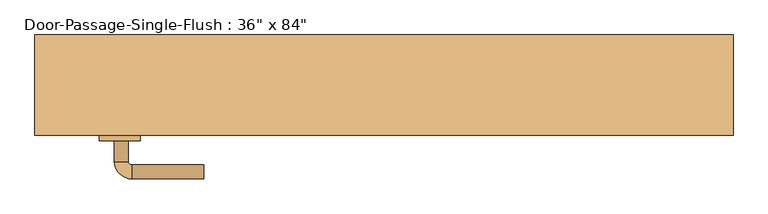
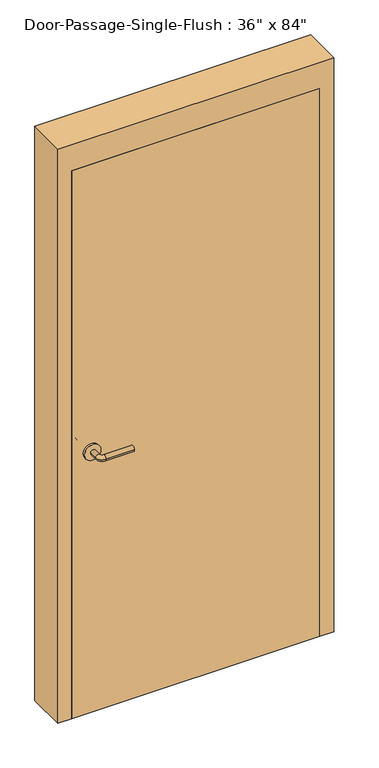
"""IFC4 building model written with IfcOpenShell, lengths in millimetres: door geometry."""

import ifcopenshell
import ifcopenshell.guid

model = None  # the IFC model being written
_history = None  # IfcOwnerHistory: only IFC2X3 demands one
_inside = {}  # id of a spatial element -> (the spatial element, [elements in it])
_under = {}  # id of a project, library or spatial element -> (it, [spatial elements below it])
_declared = {}  # id of a project -> (the project, [libraries it declares])
_typed = {}  # id of a type object -> (the type object, [elements of that type])
_made_of = {}  # id of a material, layer set ... -> (it, [elements and type objects made of it])


def new_model(schema):
    """Start an empty IFC model of exactly this schema.

    Asked for "IFC4X3", IfcOpenShell would pick the latest addendum, in which some entities
    have other attributes; the version numbers below select the first issue.
    IFC2X3 requires an IfcOwnerHistory on every rooted entity: one is made here for all.
    """
    global model, _history
    if schema == "IFC4X3":
        model = ifcopenshell.file(schema_version=(4, 3, 0, 0))
    else:
        model = ifcopenshell.file(schema=schema)
    _inside.clear()
    _under.clear()
    _declared.clear()
    _typed.clear()
    _made_of.clear()
    _history = None
    if model.schema == "IFC2X3":
        org = make("IfcOrganization", Name="unknown")
        user = make(
            "IfcPersonAndOrganization",
            ThePerson=make("IfcPerson", FamilyName="unknown"),
            TheOrganization=org,
        )
        app = make(
            "IfcApplication",
            ApplicationDeveloper=org,
            Version="unknown",
            ApplicationFullName="unknown",
            ApplicationIdentifier="unknown",
        )
        _history = make(
            "IfcOwnerHistory",
            OwningUser=user,
            OwningApplication=app,
            ChangeAction="ADDED",
            CreationDate=0,
        )
    return model


def make(cls, **values):
    """One entity of the class cls with the attributes given. An attribute that is None is left unset."""
    return model.create_entity(
        cls, **{name: value for name, value in values.items() if value is not None}
    )


def rooted(cls, **values):
    """An entity with a GlobalId (a new one), such as an element, a storey or a relation."""
    return make(cls, GlobalId=ifcopenshell.guid.new(), OwnerHistory=_history, **values)


def si_unit(unit_type, name, prefix=None):
    """IfcSIUnit, for example si_unit("LENGTHUNIT", "METRE", prefix="MILLI")."""
    return make("IfcSIUnit", UnitType=unit_type, Prefix=prefix, Name=name)


def assignment(units):
    """IfcUnitAssignment: the units of a project."""
    return None if units is None else make("IfcUnitAssignment", Units=units)


def point(xyz):
    """IfcCartesianPoint."""
    return None if xyz is None else make("IfcCartesianPoint", Coordinates=xyz)


def direction(xyz):
    """IfcDirection."""
    return None if xyz is None else make("IfcDirection", DirectionRatios=xyz)


def frame(location, z_axis=None, x_axis=None):
    """IfcAxis2Placement3D, a coordinate frame: its origin and axes. An axis left out is left unset."""
    return make(
        "IfcAxis2Placement3D",
        Location=point(location),
        Axis=direction(z_axis),
        RefDirection=direction(x_axis),
    )


def frame_2d(location, x_axis=None):
    """IfcAxis2Placement2D, a coordinate frame in the plane: its origin and x axis."""
    return make(
        "IfcAxis2Placement2D", Location=point(location), RefDirection=direction(x_axis)
    )


def origin():
    """The frame at (0, 0, 0) with its axes left unset."""
    return frame((0.0, 0.0, 0.0))


def origin_with_axes():
    """The frame at (0, 0, 0) with the z axis (0, 0, 1) and the x axis (1, 0, 0) written out."""
    return frame((0.0, 0.0, 0.0), z_axis=(0.0, 0.0, 1.0), x_axis=(1.0, 0.0, 0.0))


def place(relative_to, where):
    """IfcLocalPlacement: puts the frame where relative to a parent placement (None: the world)."""
    return make(
        "IfcLocalPlacement", PlacementRelTo=relative_to, RelativePlacement=where
    )


def context(
    kind, dimensions, precision=None, world=None, true_north=None, identifier=None
):
    """IfcGeometricRepresentationContext, for example the 3D "Model" context."""
    return make(
        "IfcGeometricRepresentationContext",
        ContextIdentifier=identifier,
        ContextType=kind,
        CoordinateSpaceDimension=dimensions,
        Precision=precision,
        WorldCoordinateSystem=world,
        TrueNorth=true_north,
    )


def project(units=None, contexts=None):
    """IfcProject with its units and contexts."""
    return rooted(
        "IfcProject",
        Name="project",
        RepresentationContexts=contexts,
        UnitsInContext=assignment(units),
    )


def spatial(cls, under=None, at=None, **own):
    """A site, building, storey or space (cls), placed at a placement, below another one or the project."""
    s = rooted(cls, ObjectPlacement=at, **own)
    if under is not None:
        _under.setdefault(under.id(), (under, []))[1].append(s)
    return s


def polyline(points):
    """IfcPolyline through the points."""
    return make("IfcPolyline", Points=[point(p) for p in points])


def circle_curve(where, radius):
    """IfcCircle in the frame where."""
    return make("IfcCircle", Position=where, Radius=radius)


def ellipse_curve(where, semi_axis1, semi_axis2):
    """IfcEllipse in the frame where."""
    return make(
        "IfcEllipse", Position=where, SemiAxis1=semi_axis1, SemiAxis2=semi_axis2
    )


def trimmed(basis, trim1, trim2, sense, master):
    """IfcTrimmedCurve: the piece of a basis curve between two trims."""
    return make(
        "IfcTrimmedCurve",
        BasisCurve=basis,
        Trim1=trim1,
        Trim2=trim2,
        SenseAgreement=sense,
        MasterRepresentation=master,
    )


def segment(curve, same_sense, transition):
    """IfcCompositeCurveSegment."""
    return make(
        "IfcCompositeCurveSegment",
        Transition=transition,
        SameSense=same_sense,
        ParentCurve=curve,
    )


def composite_curve(segments, self_intersect=None):
    """IfcCompositeCurve: segments joined end to end."""
    return make("IfcCompositeCurve", Segments=segments, SelfIntersect=self_intersect)


def outline(outer, holes=None, kind="AREA"):
    """IfcArbitraryClosedProfileDef: a profile drawn as a closed curve; with holes, ...WithVoids."""
    if holes is None:
        return make("IfcArbitraryClosedProfileDef", ProfileType=kind, OuterCurve=outer)
    return make(
        "IfcArbitraryProfileDefWithVoids",
        ProfileType=kind,
        OuterCurve=outer,
        InnerCurves=holes,
    )


def extrude(swept, where, along, depth):
    """IfcExtrudedAreaSolid: the profile swept, set in the frame where, extruded along a direction by depth."""
    return make(
        "IfcExtrudedAreaSolid",
        SweptArea=swept,
        Position=where,
        ExtrudedDirection=direction(along),
        Depth=depth,
    )


def faces_of(points, faces, orient=None, outer=None):
    """IfcFace entities. A face is a list of loops; a loop is a list of indices into points, from 0.

    orient and outer hold one flag for each loop. By default every Orientation is true, the
    first loop of a face is its IfcFaceOuterBound and the others are IfcFaceBound.
    """
    made = []
    for i, loops in enumerate(faces):
        bounds = []
        for j, loop in enumerate(loops):
            is_outer = j == 0 if outer is None else outer[i][j]
            bounds.append(
                make(
                    "IfcFaceOuterBound" if is_outer else "IfcFaceBound",
                    Bound=make("IfcPolyLoop", Polygon=[points[k] for k in loop]),
                    Orientation=True if orient is None else orient[i][j],
                )
            )
        made.append(make("IfcFace", Bounds=bounds))
    return made


def faceted_brep(points, faces, orient=None, outer=None, voids=None):
    """IfcFacetedBrep: a solid bounded by flat faces; with voids (closed shells), ...WithVoids."""
    shared = [point(p) for p in points]
    hull = make("IfcClosedShell", CfsFaces=faces_of(shared, faces, orient, outer))
    if voids is None:
        return make("IfcFacetedBrep", Outer=hull)
    return make(
        "IfcFacetedBrepWithVoids",
        Outer=hull,
        Voids=[
            make(cls, CfsFaces=faces_of(shared, fs, o, b)) for cls, fs, o, b in voids
        ],
    )


def shape(context_of_items, identifier, shape_type, items):
    """IfcShapeRepresentation: the items that make up one representation, for example the "Body"."""
    return make(
        "IfcShapeRepresentation",
        ContextOfItems=context_of_items,
        RepresentationIdentifier=identifier,
        RepresentationType=shape_type,
        Items=items,
    )


def source(mapping_origin, context_of_items, identifier, shape_type, items):
    """IfcRepresentationMap: a shape defined once, which mapped items show again and again."""
    return make(
        "IfcRepresentationMap",
        MappingOrigin=mapping_origin,
        MappedRepresentation=shape(context_of_items, identifier, shape_type, items),
    )


def transform(
    local_origin,
    x_axis=None,
    y_axis=None,
    z_axis=None,
    scale=None,
    scale2=None,
    scale3=None,
    uniform=True,
):
    """IfcCartesianTransformationOperator3D, or its non-uniform kind. x_axis, y_axis, z_axis: its Axis1, 2, 3."""
    if uniform:
        return make(
            "IfcCartesianTransformationOperator3D",
            Axis1=direction(x_axis),
            Axis2=direction(y_axis),
            LocalOrigin=point(local_origin),
            Scale=scale,
            Axis3=direction(z_axis),
        )
    return make(
        "IfcCartesianTransformationOperator3DnonUniform",
        Axis1=direction(x_axis),
        Axis2=direction(y_axis),
        LocalOrigin=point(local_origin),
        Scale=scale,
        Axis3=direction(z_axis),
        Scale2=scale2,
        Scale3=scale3,
    )


def mapped(mapping_source, mapping_target):
    """IfcMappedItem: shows the shape of a source again, moved by a transform."""
    return make(
        "IfcMappedItem", MappingSource=mapping_source, MappingTarget=mapping_target
    )


def made_of(thing, what):
    """Note that an element or type object is made of a material, layer set ...; save() writes the relation."""
    if what is not None:
        _made_of.setdefault(what.id(), (what, []))[1].append(thing)
    return thing


def element(
    cls,
    number,
    at=None,
    inside=None,
    cuts=None,
    type_object=None,
    material=None,
    context=None,
    identifier="Body",
    shape_type=None,
    held_by="IfcProductDefinitionShape",
    body=None,
    shapes=None,
    **own,
):
    """One element of the class cls, such as IfcWall. Its Tag is "e" and its number.

    at: its placement. inside: the storey or other place that contains it. cuts: it is an
    opening in that element (IfcRelVoidsElement). A single representation is given by context,
    identifier, shape_type and body (its items); several are given by shapes. held_by: the class
    of the entity that holds the representations. save() writes the other relations.
    """
    e = rooted(cls, Tag="e%d" % number, ObjectPlacement=at, **own)
    if body is not None:
        shapes = [shape(context, identifier, shape_type, body)]
    if shapes is not None:
        e.Representation = make(held_by, Representations=shapes)
    if inside is not None:
        _inside.setdefault(inside.id(), (inside, []))[1].append(e)
    if cuts is not None:
        rooted(
            "IfcRelVoidsElement", RelatingBuildingElement=cuts, RelatedOpeningElement=e
        )
    if type_object is not None:
        _typed.setdefault(type_object.id(), (type_object, []))[1].append(e)
    return made_of(e, material)


def aggregate(whole, parts):
    """IfcRelAggregates: a whole, such as a stair, and the parts it consists of."""
    return rooted("IfcRelAggregates", RelatingObject=whole, RelatedObjects=parts)


def save(model, path):
    """Write the relations noted so far, then the file.

    IfcRelAggregates (storeys below a building ...), IfcRelContainedInSpatialStructure (elements
    in a storey), IfcRelDefinesByType, IfcRelAssociatesMaterial and IfcRelDeclares: one each for
    every whole, place, type object, material and project.
    """
    for whole, parts in _under.values():
        aggregate(whole, parts)
    for where, things in _inside.values():
        rooted(
            "IfcRelContainedInSpatialStructure",
            RelatedElements=things,
            RelatingStructure=where,
        )
    for kind, things in _typed.values():
        rooted("IfcRelDefinesByType", RelatedObjects=things, RelatingType=kind)
    for what, things in _made_of.values():
        rooted("IfcRelAssociatesMaterial", RelatedObjects=things, RelatingMaterial=what)
    for by, libraries in _declared.values():
        rooted("IfcRelDeclares", RelatingContext=by, RelatedDefinitions=libraries)
    model.write(path)


def plane_surface(at):
    """IfcPlane: the flat surface through the origin of the frame at, square to its z axis."""
    return make("IfcPlane", Position=at)


def cylinder_surface(at, radius):
    """IfcCylindricalSurface: all points at the distance radius from the z axis of the frame at."""
    return make("IfcCylindricalSurface", Position=at, Radius=radius)


def revolved_surface(curve, axis_point, axis_direction):
    """IfcSurfaceOfRevolution: the curve turned about the line through axis_point along axis_direction."""
    return make(
        "IfcSurfaceOfRevolution",
        SweptCurve=make("IfcArbitraryOpenProfileDef", ProfileType="CURVE", Curve=curve),
        AxisPosition=make("IfcAxis1Placement", Location=point(axis_point), Axis=direction(axis_direction)),
    )


def advanced_brep(points, edges, surfaces, faces):
    """IfcAdvancedBrep: a solid bounded by faces that lie on surfaces and meet in shared edges.

    An edge is (start, end): straight between two places in points (the first is 0);
    or (start, end, curve); or (start, end, curve, False) where it runs against its curve.
    A face is (place in surfaces, loops), or (place, loops, False) where it looks against
    its surface's normal. A loop lists edges by number (the first is 1), with a minus sign
    where the edge is run from its end to its start. The first loop is the outer one.
    """
    corners = [point(p) for p in points]
    vertices = [make("IfcVertexPoint", VertexGeometry=c) for c in corners]
    made = []
    for start, end, *more in edges:
        made.append(
            make(
                "IfcEdgeCurve",
                EdgeStart=vertices[start],
                EdgeEnd=vertices[end],
                EdgeGeometry=more[0] if more else make("IfcPolyline", Points=[corners[start], corners[end]]),
                SameSense=more[1] if len(more) > 1 else True,
            )
        )
    hull = []
    for where, loops, *sense in faces:
        bounds = []
        for j, loop in enumerate(loops):
            ring = [make("IfcOrientedEdge", EdgeElement=made[abs(k) - 1], Orientation=k > 0) for k in loop]
            bounds.append(
                make(
                    "IfcFaceOuterBound" if j == 0 else "IfcFaceBound",
                    Bound=make("IfcEdgeLoop", EdgeList=ring),
                    Orientation=True,
                )
            )
        hull.append(make("IfcAdvancedFace", Bounds=bounds, FaceSurface=surfaces[where], SameSense=sense[0] if sense else True))
    return make("IfcAdvancedBrep", Outer=make("IfcClosedShell", CfsFaces=hull))


def door_58febf71(model_context):
    return source(origin(), model_context, "Body", "SolidModel", [
        advanced_brep(
        [(-392.190625, -76.1375, 1016.0), (-372.190625, -76.1375, 1016.0), (-392.190625, -46.1375, 1016.0), (-372.190625, -46.1375, 1016.0), (-367.190625, -41.1375, 1016.0), (-367.190625, -21.1375, 1016.0), (-262.190625, -21.1375, 1016.0), (-262.190625, -41.1375, 1016.0)],
        [
            (0, 1, circle_curve(frame((-382.190625, -76.1375, 1016.0), z_axis=(0.0, -1.0, 0.0), x_axis=(1.0, 0.0, 0.0)), 10.0)),
            (1, 0, circle_curve(frame((-382.190625, -76.1375, 1016.0), z_axis=(0.0, -1.0, 0.0), x_axis=(1.0, 0.0, 0.0)), 10.0)),
            (0, 2),
            (2, 3, circle_curve(frame((-382.190625, -46.1375, 1016.0), z_axis=(0.0, -1.0, 0.0), x_axis=(1.0, 0.0, 0.0)), 10.0)),
            (3, 1),
            (3, 2, circle_curve(frame((-382.190625, -46.1375, 1016.0), z_axis=(0.0, -1.0, 0.0), x_axis=(1.0, 0.0, 0.0)), 10.0)),
            (4, 3, circle_curve(frame((-367.190625, -46.1375, 1016.0), z_axis=(0.0, 0.0, 1.0), x_axis=(-1.0, 0.0, 0.0)), 5.0)),
            (2, 5, circle_curve(frame((-367.190625, -46.1375, 1016.0), z_axis=(0.0, 0.0, -1.0), x_axis=(-1.0, 0.0, 0.0)), 25.0)),
            (5, 4, circle_curve(frame((-367.190625, -31.1375, 1016.0), z_axis=(-1.0, 0.0, 0.0), x_axis=(0.0, -1.0, 0.0)), 10.0)),
            (4, 5, circle_curve(frame((-367.190625, -31.1375, 1016.0), z_axis=(-1.0, 0.0, 0.0), x_axis=(0.0, -1.0, 0.0)), 10.0)),
            (6, 7, circle_curve(frame((-262.190625, -31.1375, 1016.0), z_axis=(1.0, 0.0, 0.0), x_axis=(0.0, -1.0, 0.0)), 10.0)),
            (7, 6, circle_curve(frame((-262.190625, -31.1375, 1016.0), z_axis=(1.0, 0.0, 0.0), x_axis=(0.0, -1.0, 0.0)), 10.0)),
            (5, 6),
            (7, 4),
        ],
        [
            plane_surface(frame((-382.190625, -76.1375, 1016.0), z_axis=(0.0, -1.0, 0.0), x_axis=(0.0, 0.0, 1.0))),
            cylinder_surface(frame((-382.190625, -76.1375, 1016.0), z_axis=(0.0, -1.0, 0.0), x_axis=(1.0, 0.0, 0.0)), 10.0),
            revolved_surface(trimmed(ellipse_curve(frame((-382.190625, -46.1375, 1016.0), z_axis=(0.0, -1.0, 0.0), x_axis=(1.0, 0.0, 0.0)), 10.0, 10.0), [point((-392.190625, -46.1375, 1016.0))], [point((-372.190625, -46.1375, 1016.0))], True, "CARTESIAN"), (-367.190625, -46.1375, 1016.0), (0.0, 0.0, -1.0)),
            revolved_surface(trimmed(ellipse_curve(frame((-382.190625, -46.1375, 1016.0), z_axis=(0.0, -1.0, 0.0), x_axis=(1.0, 0.0, 0.0)), 10.0, 10.0), [point((-372.190625, -46.1375, 1016.0))], [point((-392.190625, -46.1375, 1016.0))], True, "CARTESIAN"), (-367.190625, -46.1375, 1016.0), (0.0, 0.0, -1.0)),
            plane_surface(frame((-262.190625, -31.1375, 1016.0), z_axis=(1.0, 0.0, 0.0), x_axis=(0.0, 0.0, 1.0))),
            cylinder_surface(frame((-367.190625, -31.1375, 1016.0), z_axis=(-1.0, 0.0, 0.0), x_axis=(0.0, -1.0, 0.0)), 10.0),
        ],
        [
            (0, [[1, 2]]),
            (1, [[-1, 3, 4, 5]]),
            (1, [[-2, -5, 6, -3]]),
            (2, [[7, -4, 8, 9]]),
            (3, [[-8, -6, -7, 10]]),
            (4, [[11, 12]]),
            (5, [[-9, 13, -12, 14]]),
            (5, [[-10, -14, -11, -13]]),
        ],
    ),
        extrude(outline(composite_curve([segment(trimmed(circle_curve(frame_2d((1016.0, -384.690625)), 30.0), [point((1016.0, -414.690625))], [point((1016.0, -354.690625))], False, "CARTESIAN"), True, "CONTINUOUS"), segment(trimmed(circle_curve(frame_2d((1016.0, -384.690625)), 30.0), [point((1016.0, -354.690625))], [point((1016.0, -414.690625))], False, "CARTESIAN"), True, "CONTINUOUS")], self_intersect=False)), frame((0.0, -84.1375, 0.0), z_axis=(0.0, 1.0, 0.0), x_axis=(0.0, 0.0, 1.0)), (0.0, 0.0, 1.0), 8.0),
        advanced_brep(
        [(-392.190625, -136.5875, 1016.0), (-372.190625, -136.5875, 1016.0), (-372.190625, -166.5875, 1016.0), (-392.190625, -166.5875, 1016.0), (-367.190625, -171.5875, 1016.0), (-367.190625, -191.5875, 1016.0), (-262.190625, -191.5875, 1016.0), (-262.190625, -171.5875, 1016.0)],
        [
            (0, 1, circle_curve(frame((-382.190625, -136.5875, 1016.0), z_axis=(0.0, 1.0, 0.0), x_axis=(1.0, 0.0, 0.0)), 10.0)),
            (1, 0, circle_curve(frame((-382.190625, -136.5875, 1016.0), z_axis=(0.0, 1.0, 0.0), x_axis=(1.0, 0.0, 0.0)), 10.0)),
            (1, 2),
            (2, 3, circle_curve(frame((-382.190625, -166.5875, 1016.0), z_axis=(0.0, 1.0, 0.0), x_axis=(1.0, 0.0, 0.0)), 10.0)),
            (3, 0),
            (3, 2, circle_curve(frame((-382.190625, -166.5875, 1016.0), z_axis=(0.0, 1.0, 0.0), x_axis=(1.0, 0.0, 0.0)), 10.0)),
            (4, 5, circle_curve(frame((-367.190625, -181.5875, 1016.0), z_axis=(-1.0, 0.0, 0.0), x_axis=(0.0, 1.0, 0.0)), 10.0)),
            (5, 3, circle_curve(frame((-367.190625, -166.5875, 1016.0), z_axis=(0.0, 0.0, -1.0), x_axis=(-1.0, 0.0, 0.0)), 25.0)),
            (2, 4, circle_curve(frame((-367.190625, -166.5875, 1016.0), z_axis=(0.0, 0.0, 1.0), x_axis=(-1.0, 0.0, 0.0)), 5.0)),
            (5, 4, circle_curve(frame((-367.190625, -181.5875, 1016.0), z_axis=(-1.0, 0.0, 0.0), x_axis=(0.0, 1.0, 0.0)), 10.0)),
            (6, 7, circle_curve(frame((-262.190625, -181.5875, 1016.0), z_axis=(1.0, 0.0, 0.0), x_axis=(0.0, 1.0, 0.0)), 10.0)),
            (7, 6, circle_curve(frame((-262.190625, -181.5875, 1016.0), z_axis=(1.0, 0.0, 0.0), x_axis=(0.0, 1.0, 0.0)), 10.0)),
            (4, 7),
            (6, 5),
        ],
        [
            plane_surface(frame((-382.190625, -136.5875, 1016.0), z_axis=(0.0, 1.0, 0.0), x_axis=(0.0, 0.0, 1.0))),
            cylinder_surface(frame((-382.190625, -136.5875, 1016.0), z_axis=(0.0, 1.0, 0.0), x_axis=(1.0, 0.0, 0.0)), 10.0),
            revolved_surface(trimmed(ellipse_curve(frame((-382.190625, -166.5875, 1016.0), z_axis=(0.0, -1.0, 0.0), x_axis=(1.0, 0.0, 0.0)), 10.0, 10.0), [point((-392.190625, -166.5875, 1016.0))], [point((-372.190625, -166.5875, 1016.0))], True, "CARTESIAN"), (-367.190625, -166.5875, 1016.0), (0.0, 0.0, -1.0)),
            revolved_surface(trimmed(ellipse_curve(frame((-382.190625, -166.5875, 1016.0), z_axis=(0.0, -1.0, 0.0), x_axis=(1.0, 0.0, 0.0)), 10.0, 10.0), [point((-372.190625, -166.5875, 1016.0))], [point((-392.190625, -166.5875, 1016.0))], True, "CARTESIAN"), (-367.190625, -166.5875, 1016.0), (0.0, 0.0, -1.0)),
            plane_surface(frame((-262.190625, -181.5875, 1016.0), z_axis=(1.0, 0.0, 0.0), x_axis=(0.0, 0.0, 1.0))),
            cylinder_surface(frame((-367.190625, -181.5875, 1016.0), z_axis=(-1.0, 0.0, 0.0), x_axis=(0.0, 1.0, 0.0)), 10.0),
        ],
        [
            (0, [[1, 2]]),
            (1, [[3, 4, 5, -2]]),
            (1, [[-5, 6, -3, -1]]),
            (2, [[7, 8, -4, 9]]),
            (3, [[10, -9, -6, -8]]),
            (4, [[11, 12]]),
            (5, [[13, -11, 14, -7]]),
            (5, [[-14, -12, -13, -10]]),
        ],
    ),
        extrude(outline(composite_curve([segment(trimmed(circle_curve(frame_2d((1016.0, -384.690625)), 30.0), [point((1016.0, -414.690625))], [point((1016.0, -354.690625))], False, "CARTESIAN"), True, "CONTINUOUS"), segment(trimmed(circle_curve(frame_2d((1016.0, -384.690625)), 30.0), [point((1016.0, -354.690625))], [point((1016.0, -414.690625))], False, "CARTESIAN"), True, "CONTINUOUS")], self_intersect=False)), frame((0.0, -136.5875, 0.0), z_axis=(0.0, 1.0, 0.0), x_axis=(0.0, 0.0, 1.0)), (0.0, 0.0, 1.0), 8.0),
        faceted_brep([(457.2, -79.375, 0.0), (441.325, -79.375, 0.0), (441.325, -31.75, 0.0), (457.2, -31.75, 0.0), (457.2, 17.4625, 0.0), (508.0, 17.4625, 0.0), (508.0, -128.5875, 0.0), (457.2, -128.5875, 0.0), (457.2, -128.5875, 2133.6), (457.2, -79.375, 2133.6), (508.0, -128.5875, 2235.2), (-508.0, -128.5875, 2235.2), (-508.0, -128.5875, 0.0), (-457.2, -128.5875, 0.0), (-457.2, -128.5875, 2133.6), (508.0, 17.4625, 2235.2), (457.2, 17.4625, 2133.6), (-457.2, 17.4625, 2133.6), (-457.2, 17.4625, 0.0), (-508.0, 17.4625, 0.0), (-508.0, 17.4625, 2235.2), (457.2, -31.75, 2133.6), (441.325, -31.75, 2117.725), (-441.325, -31.75, 2117.725), (-441.325, -31.75, 0.0), (-457.2, -31.75, 0.0), (-457.2, -31.75, 2133.6), (441.325, -79.375, 2117.725), (-457.2, -79.375, 2133.6), (-457.2, -79.375, 0.0), (-441.325, -79.375, 0.0), (-441.325, -79.375, 2117.725)], [[[0, 1, 2, 3, 4, 5, 6, 7]], [[7, 8, 9, 0]], [[6, 10, 11, 12, 13, 14, 8, 7]], [[5, 15, 10, 6]], [[4, 16, 17, 18, 19, 20, 15, 5]], [[3, 21, 16, 4]], [[2, 22, 23, 24, 25, 26, 21, 3]], [[1, 27, 22, 2]], [[0, 9, 28, 29, 30, 31, 27, 1]], [[8, 14, 28, 9]], [[16, 21, 26, 17]], [[22, 27, 31, 23]], [[12, 19, 18, 25, 24, 30, 29, 13]], [[13, 29, 28, 14]], [[11, 20, 19, 12]], [[17, 26, 25, 18]], [[23, 31, 30, 24]], [[15, 20, 11, 10]]]),
        extrude(outline(polyline([(457.2, -84.1375), (457.2, -128.5875), (-457.2, -128.5875), (-457.2, -84.1375), (457.2, -84.1375)])), origin_with_axes(), (0.0, 0.0, 1.0), 2133.6),
    ])


if __name__ == "__main__":
    model = new_model("IFC4")
    model_context = context("Model", 3, world=origin())
    ifc_project = project(units=[si_unit("LENGTHUNIT", "METRE", prefix="MILLI")], contexts=[model_context])
    site = spatial("IfcSite", under=ifc_project)
    building = spatial("IfcBuilding", under=site)
    placement = place(None, origin())
    door_shape = door_58febf71(model_context)
    element("IfcDoor", 1, ObjectType="Door-Passage-Single-Flush : 36\" x 84\"", at=placement, inside=building, context=model_context, shape_type="MappedRepresentation", body=[
        mapped(door_shape, transform((0.0, 0.0, 0.0), x_axis=(1.0, 0.0, 0.0), y_axis=(0.0, 1.0, 0.0), z_axis=(0.0, 0.0, 1.0))),
    ])
    save(model, "model.ifc")

# Revit data of these elements
# Type "Door-Passage-Single-Flush : 36\" x 84\""
#   Type Mark = "1"
#   Assembly Code = "B2030200"
#   Analytic Construction = "Wooden"
#   Thickness = 0' - 1 3/4"
#   Thermal Resistance (R) = 2.5876 (h·ft²·°F)/BTU
#   Swing Angle [instance default] = 90.00°
#   Strike Height = 3' - 4"
#   Rough Width [instance default] = 3' - 4"
#   Rough Height [instance default] = 7' - 4"
#   MF Opening Height [instance default] = 0' - 4"
#   MF Opening Width [instance default] = 0' - 4"
#   Inset Calculate [instance default] = 0' - 4"
#   Masonry Inset [instance default] = 0' - 1"
#   Height = 7' - 0"
#   Width = 3' - 0"
#   Heat Transfer Coefficient (U) = 0.3865 BTU/(h·ft²·°F)
#   Masonry Frame Depth = 0' - 5 3/4"
#   Define Thermal Properties by = 1
#   Masonry Frame [instance default] = yes
#   Function = 1
#   Dry Wall Frame [instance default] = no
#   Panel Material = Wood - Birch
#   Frame Material = Metal - Paint Finish - Grey
#   Door Handle Material = Aluminum
#   Visual Light Transmittance = 0
#   Solar Heat Gain Coefficient = 0
#   Wall Closure = (empty or 0)
# Element 1 (IfcDoor, "Door-Passage-Single-Flush : 36\" x 84\"")
#   Materials on its faces: "Aluminum", "Metal - Paint Finish - Grey", "Wood - Birch"
# Materials
#   "Wood - Birch": class "Wood", colour RGB 166 116 52, transparency 0, Cost = 0
#   "Metal - Paint Finish - Grey": class "Paint", colour RGB 104 104 104, transparency 0, Cost = 0
#   "Aluminum": class "Metal", colour RGB 247 247 247, transparency 0, Description = "Aluminum 6061", Cost = 0
